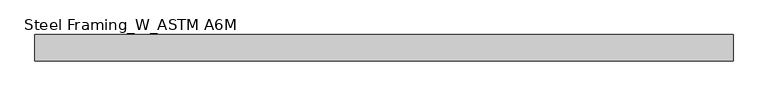
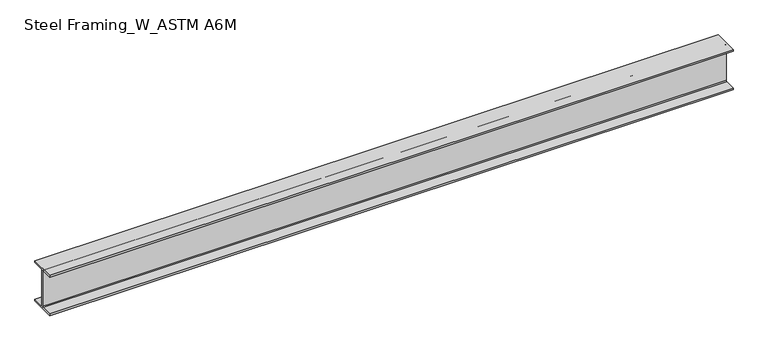
"""IFC4 building model written with IfcOpenShell, lengths in millimetres: beam geometry, Steel Framing_W_ASTM A6M : H_SB_AR_S02_W460x128_G1."""

from ifc_helpers import new_model, si_unit, point, frame, frame_2d, origin, place, context, project, spatial, polyline, circle_curve, trimmed, segment, composite_curve, outline, extrude, source, transform, mapped, element, save


def steel_framing_w_astm_a6m_5815bc2c(model_context):
    return source(origin(), model_context, "Body", "SweptSolid", [
        extrude(outline(composite_curve([segment(polyline([(141.0, -213.9), (141.0, -233.5), (-141.0, -233.5), (-141.0, -213.9), (-16.2, -213.9)]), True, "CONTINUOUS"), segment(trimmed(circle_curve(frame_2d((-16.2, -203.8)), 10.1), [point((-16.2, -213.9))], [point((-6.1, -203.8))], True, "CARTESIAN"), True, "CONTINUOUS"), segment(polyline([(-6.1, -203.8), (-6.1, 203.8)]), True, "CONTINUOUS"), segment(trimmed(circle_curve(frame_2d((-16.2, 203.8)), 10.1), [point((-6.1, 203.8))], [point((-16.2, 213.9))], True, "CARTESIAN"), True, "CONTINUOUS"), segment(polyline([(-16.2, 213.9), (-141.0, 213.9), (-141.0, 233.5), (141.0, 233.5), (141.0, 213.9), (16.2, 213.9)]), True, "CONTINUOUS"), segment(trimmed(circle_curve(frame_2d((16.2, 203.8)), 10.1), [point((16.2, 213.9))], [point((6.1, 203.8))], True, "CARTESIAN"), True, "CONTINUOUS"), segment(polyline([(6.1, 203.8), (6.1, -203.8)]), True, "CONTINUOUS"), segment(trimmed(circle_curve(frame_2d((16.2, -203.8)), 10.1), [point((6.1, -203.8))], [point((16.2, -213.9))], True, "CARTESIAN"), True, "CONTINUOUS"), segment(polyline([(16.2, -213.9), (141.0, -213.9)]), True, "CONTINUOUS")], self_intersect=False)), frame((-3753.8, 0.0, 0.0), z_axis=(1.0, 0.0, 0.0), x_axis=(0.0, 1.0, 0.0)), (0.0, 0.0, 1.0), 7507.6),
    ])


if __name__ == "__main__":
    model = new_model("IFC4")
    model_context = context("Model", 3, world=origin())
    ifc_project = project(units=[si_unit("LENGTHUNIT", "METRE", prefix="MILLI")], contexts=[model_context])
    site = spatial("IfcSite", under=ifc_project)
    building = spatial("IfcBuilding", under=site)
    placement = place(None, origin())
    steel_framing_w_astm_a6m_shape = steel_framing_w_astm_a6m_5815bc2c(model_context)
    element("IfcBeam", 1, ObjectType="Steel Framing_W_ASTM A6M : H_SB_AR_S02_W460x128_G1", at=placement, inside=building, context=model_context, shape_type="MappedRepresentation", body=[
        mapped(steel_framing_w_astm_a6m_shape, transform((0.0, 0.0, 0.0), x_axis=(1.0, 0.0, 0.0), y_axis=(0.0, 1.0, 0.0), z_axis=(0.0, 0.0, 1.0))),
    ])
    save(model, "model.ifc")

# Revit data of these elements
# Type "Steel Framing_W_ASTM A6M : H_SB_AR_S02_W460x128_G1"
#   Section Name Key = "W18x86"
#   Width = 28.2 cm
#   Web Thickness = 1.22 cm
#   Web Fillet = 1.01 cm
#   Warping Constant = 3650000.0 cm⁶
#   Torsional Moment of Inertia = 171.00 cm⁴
#   Section Area = 163.0 cm²
#   Plastic Modulus weak axis = 793.0 cm³
#   Plastic Modulus strong axis = 3050.0 cm³
#   Perimeter = 2.02 m²/m
#   Nominal Weight = 128.00 kgf/m
#   Moment of Inertia weak axis = 7280.00 cm⁴
#   Moment of Inertia strong axis = 63700.00 cm⁴
#   Height = 46.7 cm
#   Flange Thickness = 1.96 cm
#   Elastic Modulus weak axis = 518.0 cm³
#   Elastic Modulus strong axis = 2720.0 cm³
#   Centroid Vertical = 23.35 cm
#   Centroid Horizontal = 14.1 cm
#   Length [instance default] = 1500 mm
#   Structural Material [instance default] = Steel, 45-345
#   Bolt Spacing = 0
#   Assembly Code = ""
# Element 1 (IfcBeam, "Steel Framing_W_ASTM A6M : H_SB_AR_S02_W460x128_G1")
#   Materials on its faces: "Steel, 45-345"
# Materials
#   "Steel, 45-345": class "Metal", colour RGB 189 187 185, transparency 0, Description = "Steel 345 MPa", Cost = 0
